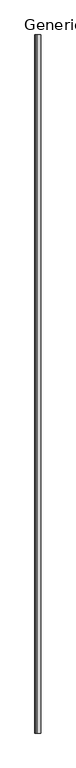
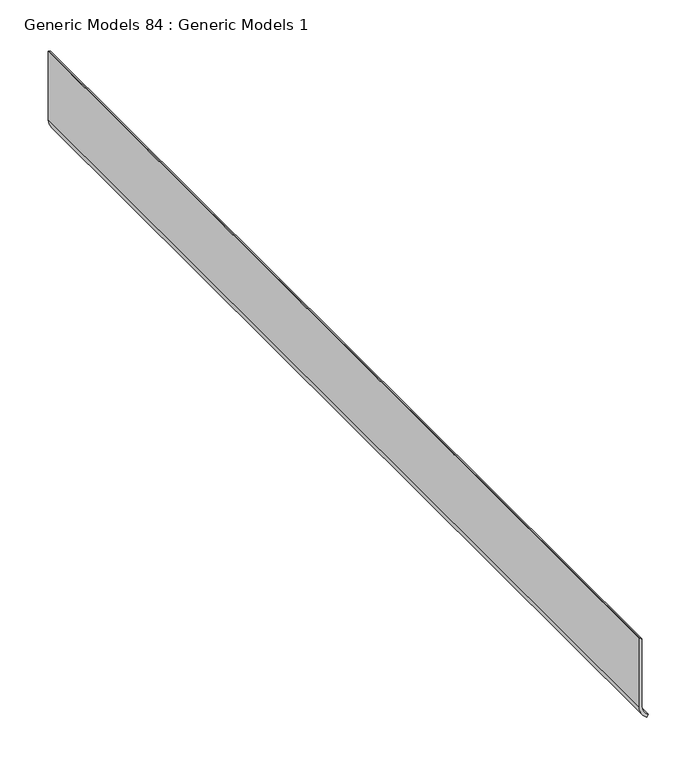
"""IFC4 building model written with IfcOpenShell, lengths in millimetres: proxy geometry, Generic Models 84 : Generic Models 1."""

import ifcopenshell
import ifcopenshell.guid

model = None  # the IFC model being written
_history = None  # IfcOwnerHistory: only IFC2X3 demands one
_inside = {}  # id of a spatial element -> (the spatial element, [elements in it])
_under = {}  # id of a project, library or spatial element -> (it, [spatial elements below it])
_declared = {}  # id of a project -> (the project, [libraries it declares])
_typed = {}  # id of a type object -> (the type object, [elements of that type])
_made_of = {}  # id of a material, layer set ... -> (it, [elements and type objects made of it])


def new_model(schema):
    """Start an empty IFC model of exactly this schema.

    Asked for "IFC4X3", IfcOpenShell would pick the latest addendum, in which some entities
    have other attributes; the version numbers below select the first issue.
    IFC2X3 requires an IfcOwnerHistory on every rooted entity: one is made here for all.
    """
    global model, _history
    if schema == "IFC4X3":
        model = ifcopenshell.file(schema_version=(4, 3, 0, 0))
    else:
        model = ifcopenshell.file(schema=schema)
    _inside.clear()
    _under.clear()
    _declared.clear()
    _typed.clear()
    _made_of.clear()
    _history = None
    if model.schema == "IFC2X3":
        org = make("IfcOrganization", Name="unknown")
        user = make(
            "IfcPersonAndOrganization",
            ThePerson=make("IfcPerson", FamilyName="unknown"),
            TheOrganization=org,
        )
        app = make(
            "IfcApplication",
            ApplicationDeveloper=org,
            Version="unknown",
            ApplicationFullName="unknown",
            ApplicationIdentifier="unknown",
        )
        _history = make(
            "IfcOwnerHistory",
            OwningUser=user,
            OwningApplication=app,
            ChangeAction="ADDED",
            CreationDate=0,
        )
    return model


def make(cls, **values):
    """One entity of the class cls with the attributes given. An attribute that is None is left unset."""
    return model.create_entity(
        cls, **{name: value for name, value in values.items() if value is not None}
    )


def rooted(cls, **values):
    """An entity with a GlobalId (a new one), such as an element, a storey or a relation."""
    return make(cls, GlobalId=ifcopenshell.guid.new(), OwnerHistory=_history, **values)


def si_unit(unit_type, name, prefix=None):
    """IfcSIUnit, for example si_unit("LENGTHUNIT", "METRE", prefix="MILLI")."""
    return make("IfcSIUnit", UnitType=unit_type, Prefix=prefix, Name=name)


def assignment(units):
    """IfcUnitAssignment: the units of a project."""
    return None if units is None else make("IfcUnitAssignment", Units=units)


def point(xyz):
    """IfcCartesianPoint."""
    return None if xyz is None else make("IfcCartesianPoint", Coordinates=xyz)


def direction(xyz):
    """IfcDirection."""
    return None if xyz is None else make("IfcDirection", DirectionRatios=xyz)


def frame(location, z_axis=None, x_axis=None):
    """IfcAxis2Placement3D, a coordinate frame: its origin and axes. An axis left out is left unset."""
    return make(
        "IfcAxis2Placement3D",
        Location=point(location),
        Axis=direction(z_axis),
        RefDirection=direction(x_axis),
    )


def frame_2d(location, x_axis=None):
    """IfcAxis2Placement2D, a coordinate frame in the plane: its origin and x axis."""
    return make(
        "IfcAxis2Placement2D", Location=point(location), RefDirection=direction(x_axis)
    )


def origin():
    """The frame at (0, 0, 0) with its axes left unset."""
    return frame((0.0, 0.0, 0.0))


def place(relative_to, where):
    """IfcLocalPlacement: puts the frame where relative to a parent placement (None: the world)."""
    return make(
        "IfcLocalPlacement", PlacementRelTo=relative_to, RelativePlacement=where
    )


def context(
    kind, dimensions, precision=None, world=None, true_north=None, identifier=None
):
    """IfcGeometricRepresentationContext, for example the 3D "Model" context."""
    return make(
        "IfcGeometricRepresentationContext",
        ContextIdentifier=identifier,
        ContextType=kind,
        CoordinateSpaceDimension=dimensions,
        Precision=precision,
        WorldCoordinateSystem=world,
        TrueNorth=true_north,
    )


def project(units=None, contexts=None):
    """IfcProject with its units and contexts."""
    return rooted(
        "IfcProject",
        Name="project",
        RepresentationContexts=contexts,
        UnitsInContext=assignment(units),
    )


def spatial(cls, under=None, at=None, **own):
    """A site, building, storey or space (cls), placed at a placement, below another one or the project."""
    s = rooted(cls, ObjectPlacement=at, **own)
    if under is not None:
        _under.setdefault(under.id(), (under, []))[1].append(s)
    return s


def polyline(points):
    """IfcPolyline through the points."""
    return make("IfcPolyline", Points=[point(p) for p in points])


def circle_curve(where, radius):
    """IfcCircle in the frame where."""
    return make("IfcCircle", Position=where, Radius=radius)


def trimmed(basis, trim1, trim2, sense, master):
    """IfcTrimmedCurve: the piece of a basis curve between two trims."""
    return make(
        "IfcTrimmedCurve",
        BasisCurve=basis,
        Trim1=trim1,
        Trim2=trim2,
        SenseAgreement=sense,
        MasterRepresentation=master,
    )


def segment(curve, same_sense, transition):
    """IfcCompositeCurveSegment."""
    return make(
        "IfcCompositeCurveSegment",
        Transition=transition,
        SameSense=same_sense,
        ParentCurve=curve,
    )


def composite_curve(segments, self_intersect=None):
    """IfcCompositeCurve: segments joined end to end."""
    return make("IfcCompositeCurve", Segments=segments, SelfIntersect=self_intersect)


def outline(outer, holes=None, kind="AREA"):
    """IfcArbitraryClosedProfileDef: a profile drawn as a closed curve; with holes, ...WithVoids."""
    if holes is None:
        return make("IfcArbitraryClosedProfileDef", ProfileType=kind, OuterCurve=outer)
    return make(
        "IfcArbitraryProfileDefWithVoids",
        ProfileType=kind,
        OuterCurve=outer,
        InnerCurves=holes,
    )


def extrude(swept, where, along, depth):
    """IfcExtrudedAreaSolid: the profile swept, set in the frame where, extruded along a direction by depth."""
    return make(
        "IfcExtrudedAreaSolid",
        SweptArea=swept,
        Position=where,
        ExtrudedDirection=direction(along),
        Depth=depth,
    )


def shape(context_of_items, identifier, shape_type, items):
    """IfcShapeRepresentation: the items that make up one representation, for example the "Body"."""
    return make(
        "IfcShapeRepresentation",
        ContextOfItems=context_of_items,
        RepresentationIdentifier=identifier,
        RepresentationType=shape_type,
        Items=items,
    )


def source(mapping_origin, context_of_items, identifier, shape_type, items):
    """IfcRepresentationMap: a shape defined once, which mapped items show again and again."""
    return make(
        "IfcRepresentationMap",
        MappingOrigin=mapping_origin,
        MappedRepresentation=shape(context_of_items, identifier, shape_type, items),
    )


def transform(
    local_origin,
    x_axis=None,
    y_axis=None,
    z_axis=None,
    scale=None,
    scale2=None,
    scale3=None,
    uniform=True,
):
    """IfcCartesianTransformationOperator3D, or its non-uniform kind. x_axis, y_axis, z_axis: its Axis1, 2, 3."""
    if uniform:
        return make(
            "IfcCartesianTransformationOperator3D",
            Axis1=direction(x_axis),
            Axis2=direction(y_axis),
            LocalOrigin=point(local_origin),
            Scale=scale,
            Axis3=direction(z_axis),
        )
    return make(
        "IfcCartesianTransformationOperator3DnonUniform",
        Axis1=direction(x_axis),
        Axis2=direction(y_axis),
        LocalOrigin=point(local_origin),
        Scale=scale,
        Axis3=direction(z_axis),
        Scale2=scale2,
        Scale3=scale3,
    )


def mapped(mapping_source, mapping_target):
    """IfcMappedItem: shows the shape of a source again, moved by a transform."""
    return make(
        "IfcMappedItem", MappingSource=mapping_source, MappingTarget=mapping_target
    )


def made_of(thing, what):
    """Note that an element or type object is made of a material, layer set ...; save() writes the relation."""
    if what is not None:
        _made_of.setdefault(what.id(), (what, []))[1].append(thing)
    return thing


def element(
    cls,
    number,
    at=None,
    inside=None,
    cuts=None,
    type_object=None,
    material=None,
    context=None,
    identifier="Body",
    shape_type=None,
    held_by="IfcProductDefinitionShape",
    body=None,
    shapes=None,
    **own,
):
    """One element of the class cls, such as IfcWall. Its Tag is "e" and its number.

    at: its placement. inside: the storey or other place that contains it. cuts: it is an
    opening in that element (IfcRelVoidsElement). A single representation is given by context,
    identifier, shape_type and body (its items); several are given by shapes. held_by: the class
    of the entity that holds the representations. save() writes the other relations.
    """
    e = rooted(cls, Tag="e%d" % number, ObjectPlacement=at, **own)
    if body is not None:
        shapes = [shape(context, identifier, shape_type, body)]
    if shapes is not None:
        e.Representation = make(held_by, Representations=shapes)
    if inside is not None:
        _inside.setdefault(inside.id(), (inside, []))[1].append(e)
    if cuts is not None:
        rooted(
            "IfcRelVoidsElement", RelatingBuildingElement=cuts, RelatedOpeningElement=e
        )
    if type_object is not None:
        _typed.setdefault(type_object.id(), (type_object, []))[1].append(e)
    return made_of(e, material)


def aggregate(whole, parts):
    """IfcRelAggregates: a whole, such as a stair, and the parts it consists of."""
    return rooted("IfcRelAggregates", RelatingObject=whole, RelatedObjects=parts)


def save(model, path):
    """Write the relations noted so far, then the file.

    IfcRelAggregates (storeys below a building ...), IfcRelContainedInSpatialStructure (elements
    in a storey), IfcRelDefinesByType, IfcRelAssociatesMaterial and IfcRelDeclares: one each for
    every whole, place, type object, material and project.
    """
    for whole, parts in _under.values():
        aggregate(whole, parts)
    for where, things in _inside.values():
        rooted(
            "IfcRelContainedInSpatialStructure",
            RelatedElements=things,
            RelatingStructure=where,
        )
    for kind, things in _typed.values():
        rooted("IfcRelDefinesByType", RelatedObjects=things, RelatingType=kind)
    for what, things in _made_of.values():
        rooted("IfcRelAssociatesMaterial", RelatedObjects=things, RelatingMaterial=what)
    for by, libraries in _declared.values():
        rooted("IfcRelDeclares", RelatingContext=by, RelatedDefinitions=libraries)
    model.write(path)


def generic_models_84_generic_models_1_3640655c(model_context):
    return source(origin(), model_context, "Body", "SweptSolid", [
        extrude(outline(composite_curve([segment(polyline([(-124.376067, 46951.7485531), (-210.5264363, 46951.7485531)]), True, "CONTINUOUS"), segment(trimmed(circle_curve(frame_2d((-210.5264363, 46969.5882499)), 17.8396968), [point((-210.5264363, 46951.7485531))], [point((-225.976067, 46960.6684015))], False, "CARTESIAN"), True, "CONTINUOUS"), segment(polyline([(-225.976067, 46960.6684015), (-223.2264363, 46962.2559015)]), True, "CONTINUOUS"), segment(trimmed(circle_curve(frame_2d((-210.5264363, 46969.5882499)), 14.6646968), [point((-223.2264363, 46962.2559015))], [point((-210.5264363, 46954.9235531))], True, "CARTESIAN"), True, "CONTINUOUS"), segment(polyline([(-210.5264363, 46954.9235531), (-126.4628688, 46954.9235531)]), True, "CONTINUOUS"), segment(trimmed(circle_curve(frame_2d((-126.4628688, 46952.8367513)), 2.0868018), [point((-126.4628688, 46954.9235531))], [point((-124.376067, 46952.8367513))], False, "CARTESIAN"), True, "CONTINUOUS"), segment(polyline([(-124.376067, 46952.8367513), (-124.376067, 46951.7485531)]), True, "CONTINUOUS")], self_intersect=False)), frame((0.0, 0.0, 0.0), z_axis=(0.0, 1.0, 0.0), x_axis=(0.0, 0.0, 1.0)), (0.0, 0.0, 1.0), 1219.2),
    ])


if __name__ == "__main__":
    model = new_model("IFC4")
    model_context = context("Model", 3, world=origin())
    ifc_project = project(units=[si_unit("LENGTHUNIT", "METRE", prefix="MILLI")], contexts=[model_context])
    site = spatial("IfcSite", under=ifc_project)
    building = spatial("IfcBuilding", under=site)
    placement = place(None, origin())
    generic_models_84_generic_models_1_shape = generic_models_84_generic_models_1_3640655c(model_context)
    element("IfcBuildingElementProxy", 1, Name="Generic Models 84 : Generic Models 1", ObjectType="Generic Models 84 : Generic Models 1", at=placement, inside=building, context=model_context, shape_type="MappedRepresentation", body=[
        mapped(generic_models_84_generic_models_1_shape, transform((0.0, 0.0, 0.0), x_axis=(1.0, 0.0, 0.0), y_axis=(0.0, 1.0, 0.0), z_axis=(0.0, 0.0, 1.0))),
    ])
    save(model, "model.ifc")

# Revit data of these elements
# Element 1 (IfcBuildingElementProxy, "Generic Models 84 : Generic Models 1")
#   Materials on its faces: "MATCH EXISTING BASE"
# Materials
#   "MATCH EXISTING BASE": class "Generic", colour RGB 120 120 120, transparency 0, Cost = 0
